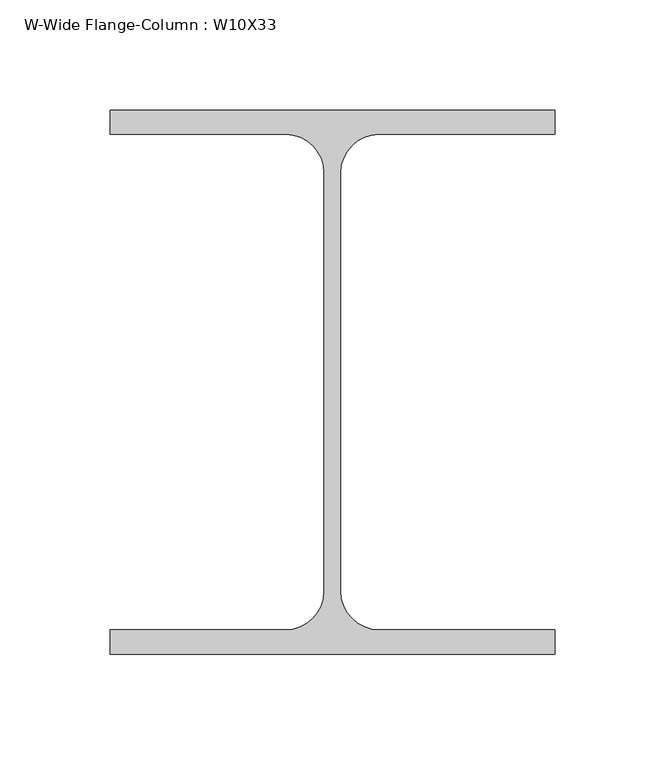
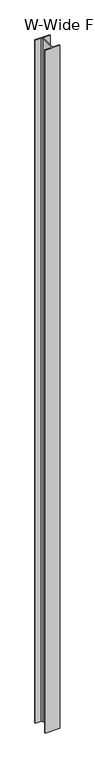
"""IFC4 building model written with IfcOpenShell, lengths in millimetres: column geometry, W-Wide Flange-Column : W10X33."""

from ifc_helpers import new_model, si_unit, point, frame, frame_2d, origin, place, context, project, spatial, polyline, circle_curve, trimmed, segment, composite_curve, outline, extrude, source, transform, mapped, element, save


def w_wide_flange_column_w10x33_e835e6bd(model_context):
    return source(origin(), model_context, "Body", "SweptSolid", [
        extrude(outline(composite_curve([segment(polyline([(101.092, 123.571), (101.092, 112.522), (21.209, 112.522)]), True, "CONTINUOUS"), segment(trimmed(circle_curve(frame_2d((21.209, 94.996)), 17.526), [point((21.209, 112.522))], [point((3.683, 94.996))], True, "CARTESIAN"), True, "CONTINUOUS"), segment(polyline([(3.683, 94.996), (3.683, -94.996)]), True, "CONTINUOUS"), segment(trimmed(circle_curve(frame_2d((21.209, -94.996)), 17.526), [point((3.683, -94.996))], [point((21.209, -112.522))], True, "CARTESIAN"), True, "CONTINUOUS"), segment(polyline([(21.209, -112.522), (101.092, -112.522), (101.092, -123.571), (-101.092, -123.571), (-101.092, -112.522), (-21.209, -112.522)]), True, "CONTINUOUS"), segment(trimmed(circle_curve(frame_2d((-21.209, -94.996)), 17.526), [point((-21.209, -112.522))], [point((-3.683, -94.996))], True, "CARTESIAN"), True, "CONTINUOUS"), segment(polyline([(-3.683, -94.996), (-3.683, 94.996)]), True, "CONTINUOUS"), segment(trimmed(circle_curve(frame_2d((-21.209, 94.996)), 17.526), [point((-3.683, 94.996))], [point((-21.209, 112.522))], True, "CARTESIAN"), True, "CONTINUOUS"), segment(polyline([(-21.209, 112.522), (-101.092, 112.522), (-101.092, 123.571), (101.092, 123.571)]), True, "CONTINUOUS")], self_intersect=False)), frame((0.0, 0.0, 17627.6), z_axis=(0.0, 0.0, 1.0), x_axis=(1.0, 0.0, 0.0)), (0.0, 0.0, 1.0), 9956.8),
    ])


if __name__ == "__main__":
    model = new_model("IFC4")
    model_context = context("Model", 3, world=origin())
    ifc_project = project(units=[si_unit("LENGTHUNIT", "METRE", prefix="MILLI")], contexts=[model_context])
    site = spatial("IfcSite", under=ifc_project)
    building = spatial("IfcBuilding", under=site)
    placement = place(None, origin())
    w_wide_flange_column_w10x33_shape = w_wide_flange_column_w10x33_e835e6bd(model_context)
    element("IfcColumn", 1, ObjectType="W-Wide Flange-Column : W10X33", at=placement, inside=building, context=model_context, shape_type="MappedRepresentation", body=[
        mapped(w_wide_flange_column_w10x33_shape, transform((0.0, 0.0, 0.0), x_axis=(1.0, 0.0, 0.0), y_axis=(0.0, 1.0, 0.0), z_axis=(0.0, 0.0, 1.0))),
    ])
    save(model, "model.ifc")

# Revit data of these elements
# Type "W-Wide Flange-Column : W10X33"
#   Assembly Code = "B10"
#   W = 33
#   bf = 0' - 7.96"
#   d = 0' - 9.73"
#   k = 0' - 1 1/8"
#   kr = 0' - 0.69"
#   tf = 0' - 0.435"
#   tw = 0' - 0.29"
#   A = 0.0674306 SF
#   Structural Material [instance default] = Steel ASTM A992
# Element 1 (IfcColumn, "W-Wide Flange-Column : W10X33")
#   Materials on its faces: "Steel ASTM A992"
# Materials
#   "Steel ASTM A992": class "Metal", colour RGB 199 199 199, transparency 0, Description = "Structural steel 50ksi", Cost = 0
